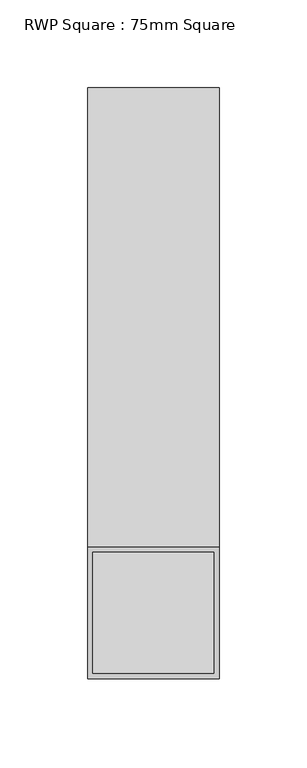
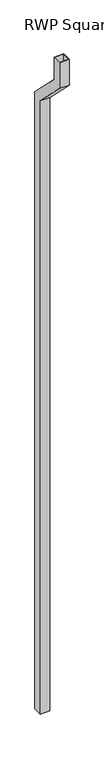
"""IFC4 building model written with IfcOpenShell, lengths in millimetres: proxy geometry, RWP Square : 75mm Square."""

import ifcopenshell
import ifcopenshell.guid

model = None  # the IFC model being written
_history = None  # IfcOwnerHistory: only IFC2X3 demands one
_inside = {}  # id of a spatial element -> (the spatial element, [elements in it])
_under = {}  # id of a project, library or spatial element -> (it, [spatial elements below it])
_declared = {}  # id of a project -> (the project, [libraries it declares])
_typed = {}  # id of a type object -> (the type object, [elements of that type])
_made_of = {}  # id of a material, layer set ... -> (it, [elements and type objects made of it])


def new_model(schema):
    """Start an empty IFC model of exactly this schema.

    Asked for "IFC4X3", IfcOpenShell would pick the latest addendum, in which some entities
    have other attributes; the version numbers below select the first issue.
    IFC2X3 requires an IfcOwnerHistory on every rooted entity: one is made here for all.
    """
    global model, _history
    if schema == "IFC4X3":
        model = ifcopenshell.file(schema_version=(4, 3, 0, 0))
    else:
        model = ifcopenshell.file(schema=schema)
    _inside.clear()
    _under.clear()
    _declared.clear()
    _typed.clear()
    _made_of.clear()
    _history = None
    if model.schema == "IFC2X3":
        org = make("IfcOrganization", Name="unknown")
        user = make(
            "IfcPersonAndOrganization",
            ThePerson=make("IfcPerson", FamilyName="unknown"),
            TheOrganization=org,
        )
        app = make(
            "IfcApplication",
            ApplicationDeveloper=org,
            Version="unknown",
            ApplicationFullName="unknown",
            ApplicationIdentifier="unknown",
        )
        _history = make(
            "IfcOwnerHistory",
            OwningUser=user,
            OwningApplication=app,
            ChangeAction="ADDED",
            CreationDate=0,
        )
    return model


def make(cls, **values):
    """One entity of the class cls with the attributes given. An attribute that is None is left unset."""
    return model.create_entity(
        cls, **{name: value for name, value in values.items() if value is not None}
    )


def rooted(cls, **values):
    """An entity with a GlobalId (a new one), such as an element, a storey or a relation."""
    return make(cls, GlobalId=ifcopenshell.guid.new(), OwnerHistory=_history, **values)


def si_unit(unit_type, name, prefix=None):
    """IfcSIUnit, for example si_unit("LENGTHUNIT", "METRE", prefix="MILLI")."""
    return make("IfcSIUnit", UnitType=unit_type, Prefix=prefix, Name=name)


def assignment(units):
    """IfcUnitAssignment: the units of a project."""
    return None if units is None else make("IfcUnitAssignment", Units=units)


def point(xyz):
    """IfcCartesianPoint."""
    return None if xyz is None else make("IfcCartesianPoint", Coordinates=xyz)


def direction(xyz):
    """IfcDirection."""
    return None if xyz is None else make("IfcDirection", DirectionRatios=xyz)


def frame(location, z_axis=None, x_axis=None):
    """IfcAxis2Placement3D, a coordinate frame: its origin and axes. An axis left out is left unset."""
    return make(
        "IfcAxis2Placement3D",
        Location=point(location),
        Axis=direction(z_axis),
        RefDirection=direction(x_axis),
    )


def origin():
    """The frame at (0, 0, 0) with its axes left unset."""
    return frame((0.0, 0.0, 0.0))


def place(relative_to, where):
    """IfcLocalPlacement: puts the frame where relative to a parent placement (None: the world)."""
    return make(
        "IfcLocalPlacement", PlacementRelTo=relative_to, RelativePlacement=where
    )


def context(
    kind, dimensions, precision=None, world=None, true_north=None, identifier=None
):
    """IfcGeometricRepresentationContext, for example the 3D "Model" context."""
    return make(
        "IfcGeometricRepresentationContext",
        ContextIdentifier=identifier,
        ContextType=kind,
        CoordinateSpaceDimension=dimensions,
        Precision=precision,
        WorldCoordinateSystem=world,
        TrueNorth=true_north,
    )


def project(units=None, contexts=None):
    """IfcProject with its units and contexts."""
    return rooted(
        "IfcProject",
        Name="project",
        RepresentationContexts=contexts,
        UnitsInContext=assignment(units),
    )


def spatial(cls, under=None, at=None, **own):
    """A site, building, storey or space (cls), placed at a placement, below another one or the project."""
    s = rooted(cls, ObjectPlacement=at, **own)
    if under is not None:
        _under.setdefault(under.id(), (under, []))[1].append(s)
    return s


def faces_of(points, faces, orient=None, outer=None):
    """IfcFace entities. A face is a list of loops; a loop is a list of indices into points, from 0.

    orient and outer hold one flag for each loop. By default every Orientation is true, the
    first loop of a face is its IfcFaceOuterBound and the others are IfcFaceBound.
    """
    made = []
    for i, loops in enumerate(faces):
        bounds = []
        for j, loop in enumerate(loops):
            is_outer = j == 0 if outer is None else outer[i][j]
            bounds.append(
                make(
                    "IfcFaceOuterBound" if is_outer else "IfcFaceBound",
                    Bound=make("IfcPolyLoop", Polygon=[points[k] for k in loop]),
                    Orientation=True if orient is None else orient[i][j],
                )
            )
        made.append(make("IfcFace", Bounds=bounds))
    return made


def faceted_brep(points, faces, orient=None, outer=None, voids=None):
    """IfcFacetedBrep: a solid bounded by flat faces; with voids (closed shells), ...WithVoids."""
    shared = [point(p) for p in points]
    hull = make("IfcClosedShell", CfsFaces=faces_of(shared, faces, orient, outer))
    if voids is None:
        return make("IfcFacetedBrep", Outer=hull)
    return make(
        "IfcFacetedBrepWithVoids",
        Outer=hull,
        Voids=[
            make(cls, CfsFaces=faces_of(shared, fs, o, b)) for cls, fs, o, b in voids
        ],
    )


def shape(context_of_items, identifier, shape_type, items):
    """IfcShapeRepresentation: the items that make up one representation, for example the "Body"."""
    return make(
        "IfcShapeRepresentation",
        ContextOfItems=context_of_items,
        RepresentationIdentifier=identifier,
        RepresentationType=shape_type,
        Items=items,
    )


def source(mapping_origin, context_of_items, identifier, shape_type, items):
    """IfcRepresentationMap: a shape defined once, which mapped items show again and again."""
    return make(
        "IfcRepresentationMap",
        MappingOrigin=mapping_origin,
        MappedRepresentation=shape(context_of_items, identifier, shape_type, items),
    )


def transform(
    local_origin,
    x_axis=None,
    y_axis=None,
    z_axis=None,
    scale=None,
    scale2=None,
    scale3=None,
    uniform=True,
):
    """IfcCartesianTransformationOperator3D, or its non-uniform kind. x_axis, y_axis, z_axis: its Axis1, 2, 3."""
    if uniform:
        return make(
            "IfcCartesianTransformationOperator3D",
            Axis1=direction(x_axis),
            Axis2=direction(y_axis),
            LocalOrigin=point(local_origin),
            Scale=scale,
            Axis3=direction(z_axis),
        )
    return make(
        "IfcCartesianTransformationOperator3DnonUniform",
        Axis1=direction(x_axis),
        Axis2=direction(y_axis),
        LocalOrigin=point(local_origin),
        Scale=scale,
        Axis3=direction(z_axis),
        Scale2=scale2,
        Scale3=scale3,
    )


def mapped(mapping_source, mapping_target):
    """IfcMappedItem: shows the shape of a source again, moved by a transform."""
    return make(
        "IfcMappedItem", MappingSource=mapping_source, MappingTarget=mapping_target
    )


def made_of(thing, what):
    """Note that an element or type object is made of a material, layer set ...; save() writes the relation."""
    if what is not None:
        _made_of.setdefault(what.id(), (what, []))[1].append(thing)
    return thing


def element(
    cls,
    number,
    at=None,
    inside=None,
    cuts=None,
    type_object=None,
    material=None,
    context=None,
    identifier="Body",
    shape_type=None,
    held_by="IfcProductDefinitionShape",
    body=None,
    shapes=None,
    **own,
):
    """One element of the class cls, such as IfcWall. Its Tag is "e" and its number.

    at: its placement. inside: the storey or other place that contains it. cuts: it is an
    opening in that element (IfcRelVoidsElement). A single representation is given by context,
    identifier, shape_type and body (its items); several are given by shapes. held_by: the class
    of the entity that holds the representations. save() writes the other relations.
    """
    e = rooted(cls, Tag="e%d" % number, ObjectPlacement=at, **own)
    if body is not None:
        shapes = [shape(context, identifier, shape_type, body)]
    if shapes is not None:
        e.Representation = make(held_by, Representations=shapes)
    if inside is not None:
        _inside.setdefault(inside.id(), (inside, []))[1].append(e)
    if cuts is not None:
        rooted(
            "IfcRelVoidsElement", RelatingBuildingElement=cuts, RelatedOpeningElement=e
        )
    if type_object is not None:
        _typed.setdefault(type_object.id(), (type_object, []))[1].append(e)
    return made_of(e, material)


def aggregate(whole, parts):
    """IfcRelAggregates: a whole, such as a stair, and the parts it consists of."""
    return rooted("IfcRelAggregates", RelatingObject=whole, RelatedObjects=parts)


def save(model, path):
    """Write the relations noted so far, then the file.

    IfcRelAggregates (storeys below a building ...), IfcRelContainedInSpatialStructure (elements
    in a storey), IfcRelDefinesByType, IfcRelAssociatesMaterial and IfcRelDeclares: one each for
    every whole, place, type object, material and project.
    """
    for whole, parts in _under.values():
        aggregate(whole, parts)
    for where, things in _inside.values():
        rooted(
            "IfcRelContainedInSpatialStructure",
            RelatedElements=things,
            RelatingStructure=where,
        )
    for kind, things in _typed.values():
        rooted("IfcRelDefinesByType", RelatedObjects=things, RelatingType=kind)
    for what, things in _made_of.values():
        rooted("IfcRelAssociatesMaterial", RelatedObjects=things, RelatingMaterial=what)
    for by, libraries in _declared.values():
        rooted("IfcRelDeclares", RelatingContext=by, RelatedDefinitions=libraries)
    model.write(path)


def rwp_square_75mm_square_53b424de(model_context):
    return source(origin(), model_context, "Body", "Brep", [
        faceted_brep([(37.5, -0.5, 0.0), (37.5, -75.5, 0.0), (-37.5, -75.5, 0.0), (-37.5, -0.5, 0.0), (34.5, -3.5, 0.0), (-34.5, -3.5, 0.0), (-34.5, -72.5, 0.0), (34.5, -72.5, 0.0), (-37.5, -0.5, 5153.5330086), (37.5, -0.5, 5153.5330086), (-37.5, -75.5, 5122.4669914), (-37.5, -337.5, 5384.4669914), (-37.5, -337.5, 5600.0), (-37.5, -262.5, 5600.0), (-37.5, -262.5, 5415.5330086), (37.5, -75.5, 5122.4669914), (37.5, -262.5, 5415.5330086), (37.5, -262.5, 5600.0), (37.5, -337.5, 5600.0), (37.5, -337.5, 5384.4669914), (34.5, -72.5, 5123.7096321), (34.5, -334.5, 5385.7096321), (34.5, -334.5, 5600.0), (34.5, -265.5, 5600.0), (34.5, -265.5, 5414.2903679), (34.5, -3.5, 5152.2903679), (-34.5, -72.5, 5123.7096321), (-34.5, -3.5, 5152.2903679), (-34.5, -265.5, 5414.2903679), (-34.5, -265.5, 5600.0), (-34.5, -334.5, 5600.0), (-34.5, -334.5, 5385.7096321)], [[[0, 1, 2, 3], [4, 5, 6, 7]], [[3, 8, 9, 0]], [[2, 10, 11, 12, 13, 14, 8, 3]], [[1, 15, 10, 2]], [[0, 9, 16, 17, 18, 19, 15, 1]], [[7, 20, 21, 22, 23, 24, 25, 4]], [[6, 26, 20, 7]], [[5, 27, 28, 29, 30, 31, 26, 6]], [[4, 25, 27, 5]], [[8, 14, 16, 9]], [[15, 19, 11, 10]], [[26, 31, 21, 20]], [[25, 24, 28, 27]], [[17, 13, 12, 18], [23, 22, 30, 29]], [[14, 13, 17, 16]], [[19, 18, 12, 11]], [[31, 30, 22, 21]], [[24, 23, 29, 28]]]),
    ])


if __name__ == "__main__":
    model = new_model("IFC4")
    model_context = context("Model", 3, world=origin())
    ifc_project = project(units=[si_unit("LENGTHUNIT", "METRE", prefix="MILLI")], contexts=[model_context])
    site = spatial("IfcSite", under=ifc_project)
    building = spatial("IfcBuilding", under=site)
    placement = place(None, origin())
    rwp_square_75mm_square_shape = rwp_square_75mm_square_53b424de(model_context)
    element("IfcBuildingElementProxy", 1, Name="RWP Square : 75mm Square", ObjectType="RWP Square : 75mm Square", at=placement, inside=building, context=model_context, shape_type="MappedRepresentation", body=[
        mapped(rwp_square_75mm_square_shape, transform((0.0, 0.0, 0.0), x_axis=(1.0, 0.0, 0.0), y_axis=(0.0, 1.0, 0.0), z_axis=(0.0, 0.0, 1.0))),
    ])
    save(model, "model.ifc")

# Revit data of these elements
# Type "RWP Square : 75mm Square"
#   Keynote = "R"
#   RWP Width = 75 mm
#   RWP Wall Thickness = 3 mm
#   RWP Depth = 75 mm
#   Offset Top = 300 mm
#   Offset Base = 38 mm
#   Height of RWP [instance default] = 5000 mm
#   Head Splayed Depth = 262 mm
#   Head Depth = 200 mm
#   Material RWP = Plastic - White
#   Default Elevation = 0
# Element 1 (IfcBuildingElementProxy, "RWP Square : 75mm Square")
#   Height of RWP = 5600 mm
#   Materials on its faces: "Plastic - White"
# Materials
#   "Plastic - White": class "Plastic", colour RGB 249 249 249, transparency 0
